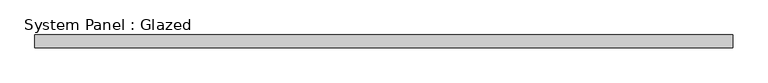
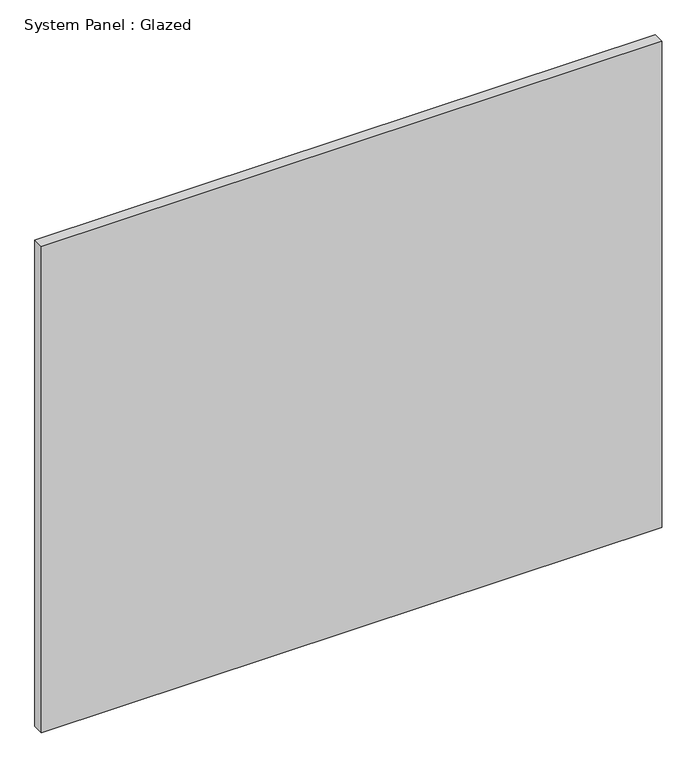
"""IFC4 building model written with IfcOpenShell, lengths in millimetres: plate geometry, System Panel : Glazed."""

from ifc_helpers import new_model, si_unit, origin, origin_with_axes, place, context, project, spatial, polyline, outline, extrude, source, transform, mapped, element, save


def system_panel_glazed_88b4eb2b(model_context):
    return source(origin(), model_context, "Body", "SweptSolid", [
        extrude(outline(polyline([(697.4416668, 19.05), (-697.4416668, 19.05), (-697.4416668, 44.45), (697.4416668, 44.45), (697.4416668, 19.05)])), origin_with_axes(), (0.0, 0.0, 1.0), 1155.7),
    ])


if __name__ == "__main__":
    model = new_model("IFC4")
    model_context = context("Model", 3, world=origin())
    ifc_project = project(units=[si_unit("LENGTHUNIT", "METRE", prefix="MILLI")], contexts=[model_context])
    site = spatial("IfcSite", under=ifc_project)
    building = spatial("IfcBuilding", under=site)
    placement = place(None, origin())
    system_panel_glazed_shape = system_panel_glazed_88b4eb2b(model_context)
    element("IfcPlate", 1, ObjectType="System Panel : Glazed", at=placement, inside=building, context=model_context, shape_type="MappedRepresentation", body=[
        mapped(system_panel_glazed_shape, transform((0.0, 0.0, 0.0), x_axis=(1.0, 0.0, 0.0), y_axis=(0.0, 1.0, 0.0), z_axis=(0.0, 0.0, 1.0))),
    ])
    save(model, "model.ifc")

# Revit data of these elements
# Type "System Panel : Glazed"
#   Construction Type Id = "GSP4R"
#   Analytic Construction = "1/8 in Pilkington single glazing"
#   Visual Light Transmittance = 0.9
#   Solar Heat Gain Coefficient = 0.86
#   Heat Transfer Coefficient (U) = 1.18115 BTU/(h·ft²·°F)
#   Define Thermal Properties by = 1
# Element 1 (IfcPlate, "System Panel : Glazed")
#   Materials on its faces: "Glass"
# Materials
#   "Glass": class "Glass", colour RGB 0 128 192, transparency 0.75, Description = "Soda Lime Glass", Cost = 0
